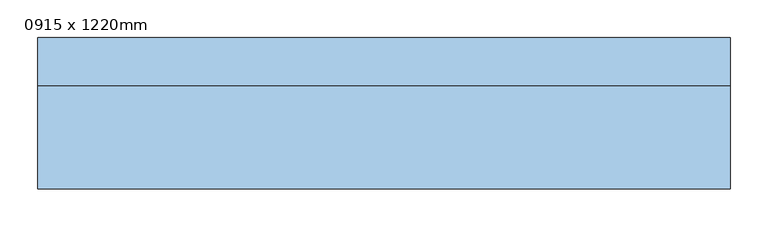
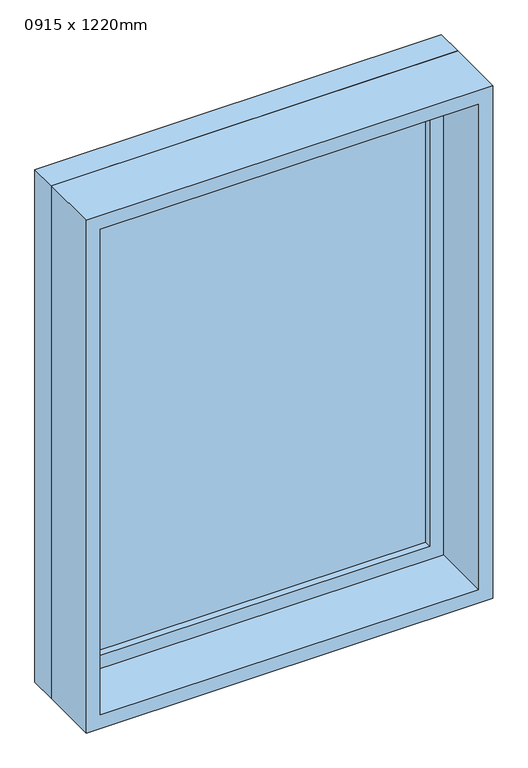
"""IFC4 building model written with IfcOpenShell, lengths in millimetres: window geometry, 固定 : 0915 x 1220mm."""

from ifc_helpers import new_model, si_unit, frame, origin, place, context, project, spatial, polyline, outline, extrude, source, transform, mapped, element, save


def window_0915_x_1220mm_488fb2fb(model_context):
    return source(origin(), model_context, "Body", "SweptSolid", [
        extrude(outline(polyline([(-394.5, 78.0), (394.5, 78.0), (394.5, 66.0), (-394.5, 66.0), (-394.5, 78.0)])), frame((0.0, 0.0, 978.0), z_axis=(0.0, 0.0, 1.0), x_axis=(1.0, 0.0, 0.0)), (0.0, 0.0, 1.0), 1094.0),
        extrude(outline(polyline([(2116.0, -438.5), (934.0, -438.5), (934.0, 438.5), (2116.0, 438.5), (2116.0, -438.5)]), holes=[polyline([(2072.0, -394.5), (2072.0, 394.5), (978.0, 394.5), (978.0, -394.5), (2072.0, -394.5)])]), frame((0.0, 50.0, 0.0), z_axis=(0.0, 1.0, 0.0), x_axis=(0.0, 0.0, 1.0)), (0.0, 0.0, 1.0), 44.0),
        extrude(outline(polyline([(2135.0, -457.5), (915.0, -457.5), (915.0, 457.5), (2135.0, 457.5), (2135.0, -457.5)]), holes=[polyline([(2116.0, -438.5), (2116.0, 438.5), (934.0, 438.5), (934.0, -438.5), (2116.0, -438.5)])]), frame((0.0, 50.0, 0.0), z_axis=(0.0, 1.0, 0.0), x_axis=(0.0, 0.0, 1.0)), (0.0, 0.0, 1.0), 63.0),
        extrude(outline(polyline([(2135.0, -457.5), (915.0, -457.5), (915.0, 457.5), (2135.0, 457.5), (2135.0, -457.5)]), holes=[polyline([(2103.0, -425.5), (2103.0, 425.5), (947.0, 425.5), (947.0, -425.5), (2103.0, -425.5)])]), frame((0.0, -87.0, 0.0), z_axis=(0.0, 1.0, 0.0), x_axis=(0.0, 0.0, 1.0)), (0.0, 0.0, 1.0), 137.0),
    ])


if __name__ == "__main__":
    model = new_model("IFC4")
    model_context = context("Model", 3, world=origin())
    ifc_project = project(units=[si_unit("LENGTHUNIT", "METRE", prefix="MILLI")], contexts=[model_context])
    site = spatial("IfcSite", under=ifc_project)
    building = spatial("IfcBuilding", under=site)
    placement = place(None, origin())
    window_0915_x_1220mm_shape = window_0915_x_1220mm_488fb2fb(model_context)
    element("IfcWindow", 1, ObjectType="固定 : 0915 x 1220mm", at=placement, inside=building, context=model_context, shape_type="MappedRepresentation", body=[
        mapped(window_0915_x_1220mm_shape, transform((0.0, 0.0, 0.0), x_axis=(1.0, 0.0, 0.0), y_axis=(0.0, 1.0, 0.0), z_axis=(0.0, 0.0, 1.0))),
    ])
    save(model, "model.ifc")

# Revit data of these elements
# Type "固定 : 0915 x 1220mm"
#   Type Mark = "15"
#   Construction Type Id = "GSP4R"
#   Analytic Construction = "1/8 英寸 Pilkington 单层玻璃"
#   Visual Light Transmittance = 0.9
#   Solar Heat Gain Coefficient = 0.78
#   Heat Transfer Coefficient (U) = 3.6886 W/(m²·K)
#   Height = 1220 mm
#   默认窗台高度 = 915 mm
#   Width = 915 mm
#   窗嵌入 = 19 mm
#   框架外部材质 = 窗扇
#   框架内部材质 = 窗扇
#   玻璃嵌板材质 = 玻璃
#   窗扇 = 窗扇
#   Wall Closure = (empty or 0)
# Element 1 (IfcWindow, "固定 : 0915 x 1220mm")
#   Materials on its faces: "窗扇", "玻璃"
# Materials
#   "窗扇": class "木质", colour RGB 224 178 126, transparency 0, Cost = 0
#   "玻璃": class "玻璃", colour RGB 0 128 192, transparency 0.9, Description = "钠钙玻璃", Cost = 0
